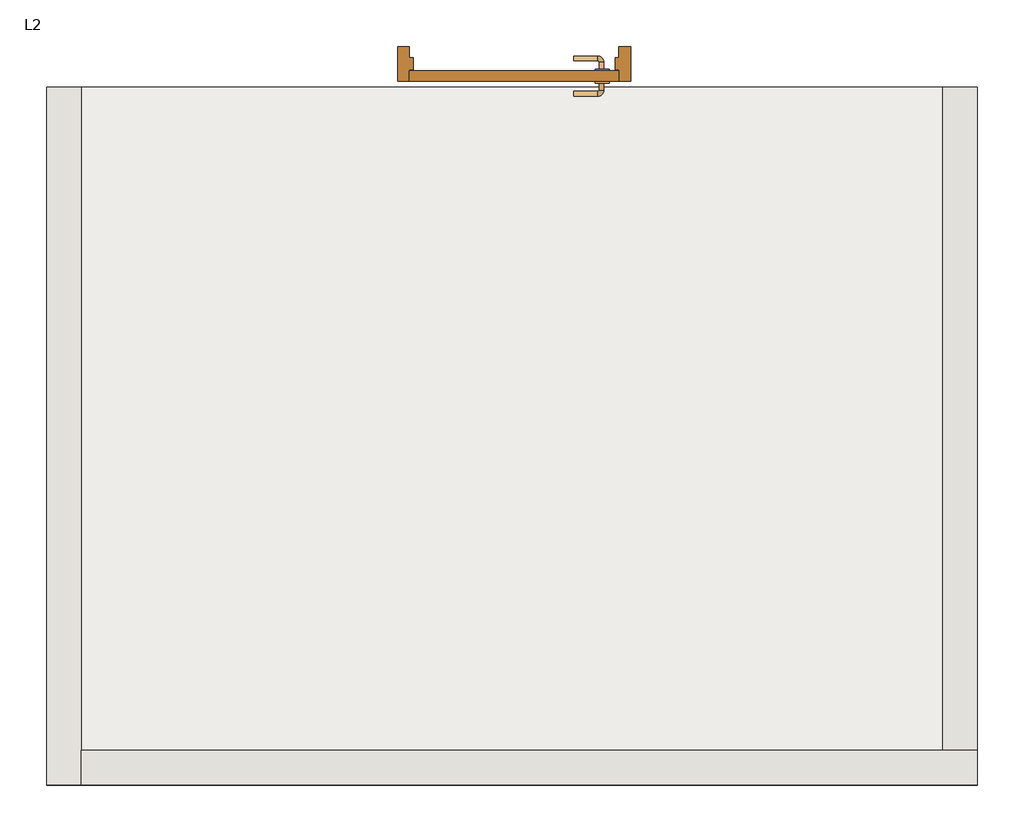
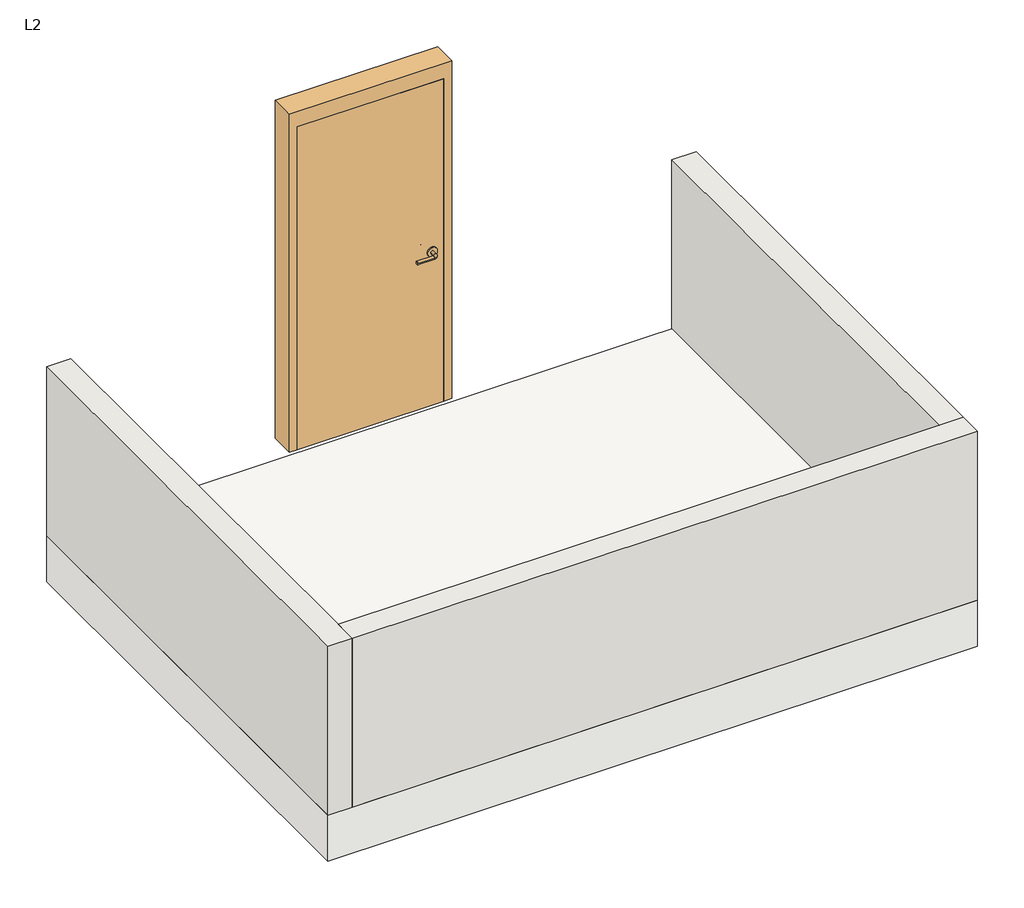
# One storey: 3 walls, 1 door, 1 slab.
"""IFC4 building model written with IfcOpenShell, lengths in millimetres."""

import ifcopenshell
import ifcopenshell.guid

model = None  # the IFC model being written
_history = None  # IfcOwnerHistory: only IFC2X3 demands one
_inside = {}  # id of a spatial element -> (the spatial element, [elements in it])
_under = {}  # id of a project, library or spatial element -> (it, [spatial elements below it])
_declared = {}  # id of a project -> (the project, [libraries it declares])
_typed = {}  # id of a type object -> (the type object, [elements of that type])
_made_of = {}  # id of a material, layer set ... -> (it, [elements and type objects made of it])


def new_model(schema):
    """Start an empty IFC model of exactly this schema.

    Asked for "IFC4X3", IfcOpenShell would pick the latest addendum, in which some entities
    have other attributes; the version numbers below select the first issue.
    IFC2X3 requires an IfcOwnerHistory on every rooted entity: one is made here for all.
    """
    global model, _history
    if schema == "IFC4X3":
        model = ifcopenshell.file(schema_version=(4, 3, 0, 0))
    else:
        model = ifcopenshell.file(schema=schema)
    _inside.clear()
    _under.clear()
    _declared.clear()
    _typed.clear()
    _made_of.clear()
    _history = None
    if model.schema == "IFC2X3":
        org = make("IfcOrganization", Name="unknown")
        user = make(
            "IfcPersonAndOrganization",
            ThePerson=make("IfcPerson", FamilyName="unknown"),
            TheOrganization=org,
        )
        app = make(
            "IfcApplication",
            ApplicationDeveloper=org,
            Version="unknown",
            ApplicationFullName="unknown",
            ApplicationIdentifier="unknown",
        )
        _history = make(
            "IfcOwnerHistory",
            OwningUser=user,
            OwningApplication=app,
            ChangeAction="ADDED",
            CreationDate=0,
        )
    return model


def make(cls, **values):
    """One entity of the class cls with the attributes given. An attribute that is None is left unset."""
    return model.create_entity(
        cls, **{name: value for name, value in values.items() if value is not None}
    )


def rooted(cls, **values):
    """An entity with a GlobalId (a new one), such as an element, a storey or a relation."""
    return make(cls, GlobalId=ifcopenshell.guid.new(), OwnerHistory=_history, **values)


def si_unit(unit_type, name, prefix=None):
    """IfcSIUnit, for example si_unit("LENGTHUNIT", "METRE", prefix="MILLI")."""
    return make("IfcSIUnit", UnitType=unit_type, Prefix=prefix, Name=name)


def assignment(units):
    """IfcUnitAssignment: the units of a project."""
    return None if units is None else make("IfcUnitAssignment", Units=units)


def point(xyz):
    """IfcCartesianPoint."""
    return None if xyz is None else make("IfcCartesianPoint", Coordinates=xyz)


def direction(xyz):
    """IfcDirection."""
    return None if xyz is None else make("IfcDirection", DirectionRatios=xyz)


def frame(location, z_axis=None, x_axis=None):
    """IfcAxis2Placement3D, a coordinate frame: its origin and axes. An axis left out is left unset."""
    return make(
        "IfcAxis2Placement3D",
        Location=point(location),
        Axis=direction(z_axis),
        RefDirection=direction(x_axis),
    )


def frame_2d(location, x_axis=None):
    """IfcAxis2Placement2D, a coordinate frame in the plane: its origin and x axis."""
    return make(
        "IfcAxis2Placement2D", Location=point(location), RefDirection=direction(x_axis)
    )


def origin():
    """The frame at (0, 0, 0) with its axes left unset."""
    return frame((0.0, 0.0, 0.0))


def origin_with_axes():
    """The frame at (0, 0, 0) with the z axis (0, 0, 1) and the x axis (1, 0, 0) written out."""
    return frame((0.0, 0.0, 0.0), z_axis=(0.0, 0.0, 1.0), x_axis=(1.0, 0.0, 0.0))


def place(relative_to, where):
    """IfcLocalPlacement: puts the frame where relative to a parent placement (None: the world)."""
    return make(
        "IfcLocalPlacement", PlacementRelTo=relative_to, RelativePlacement=where
    )


def context(
    kind, dimensions, precision=None, world=None, true_north=None, identifier=None
):
    """IfcGeometricRepresentationContext, for example the 3D "Model" context."""
    return make(
        "IfcGeometricRepresentationContext",
        ContextIdentifier=identifier,
        ContextType=kind,
        CoordinateSpaceDimension=dimensions,
        Precision=precision,
        WorldCoordinateSystem=world,
        TrueNorth=true_north,
    )


def project(units=None, contexts=None):
    """IfcProject with its units and contexts."""
    return rooted(
        "IfcProject",
        Name="project",
        RepresentationContexts=contexts,
        UnitsInContext=assignment(units),
    )


def spatial(cls, under=None, at=None, **own):
    """A site, building, storey or space (cls), placed at a placement, below another one or the project."""
    s = rooted(cls, ObjectPlacement=at, **own)
    if under is not None:
        _under.setdefault(under.id(), (under, []))[1].append(s)
    return s


def polyline(points):
    """IfcPolyline through the points."""
    return make("IfcPolyline", Points=[point(p) for p in points])


def circle_curve(where, radius):
    """IfcCircle in the frame where."""
    return make("IfcCircle", Position=where, Radius=radius)


def ellipse_curve(where, semi_axis1, semi_axis2):
    """IfcEllipse in the frame where."""
    return make(
        "IfcEllipse", Position=where, SemiAxis1=semi_axis1, SemiAxis2=semi_axis2
    )


def trimmed(basis, trim1, trim2, sense, master):
    """IfcTrimmedCurve: the piece of a basis curve between two trims."""
    return make(
        "IfcTrimmedCurve",
        BasisCurve=basis,
        Trim1=trim1,
        Trim2=trim2,
        SenseAgreement=sense,
        MasterRepresentation=master,
    )


def segment(curve, same_sense, transition):
    """IfcCompositeCurveSegment."""
    return make(
        "IfcCompositeCurveSegment",
        Transition=transition,
        SameSense=same_sense,
        ParentCurve=curve,
    )


def composite_curve(segments, self_intersect=None):
    """IfcCompositeCurve: segments joined end to end."""
    return make("IfcCompositeCurve", Segments=segments, SelfIntersect=self_intersect)


def outline(outer, holes=None, kind="AREA"):
    """IfcArbitraryClosedProfileDef: a profile drawn as a closed curve; with holes, ...WithVoids."""
    if holes is None:
        return make("IfcArbitraryClosedProfileDef", ProfileType=kind, OuterCurve=outer)
    return make(
        "IfcArbitraryProfileDefWithVoids",
        ProfileType=kind,
        OuterCurve=outer,
        InnerCurves=holes,
    )


def extrude(swept, where, along, depth):
    """IfcExtrudedAreaSolid: the profile swept, set in the frame where, extruded along a direction by depth."""
    return make(
        "IfcExtrudedAreaSolid",
        SweptArea=swept,
        Position=where,
        ExtrudedDirection=direction(along),
        Depth=depth,
    )


def faces_of(points, faces, orient=None, outer=None):
    """IfcFace entities. A face is a list of loops; a loop is a list of indices into points, from 0.

    orient and outer hold one flag for each loop. By default every Orientation is true, the
    first loop of a face is its IfcFaceOuterBound and the others are IfcFaceBound.
    """
    made = []
    for i, loops in enumerate(faces):
        bounds = []
        for j, loop in enumerate(loops):
            is_outer = j == 0 if outer is None else outer[i][j]
            bounds.append(
                make(
                    "IfcFaceOuterBound" if is_outer else "IfcFaceBound",
                    Bound=make("IfcPolyLoop", Polygon=[points[k] for k in loop]),
                    Orientation=True if orient is None else orient[i][j],
                )
            )
        made.append(make("IfcFace", Bounds=bounds))
    return made


def faceted_brep(points, faces, orient=None, outer=None, voids=None):
    """IfcFacetedBrep: a solid bounded by flat faces; with voids (closed shells), ...WithVoids."""
    shared = [point(p) for p in points]
    hull = make("IfcClosedShell", CfsFaces=faces_of(shared, faces, orient, outer))
    if voids is None:
        return make("IfcFacetedBrep", Outer=hull)
    return make(
        "IfcFacetedBrepWithVoids",
        Outer=hull,
        Voids=[
            make(cls, CfsFaces=faces_of(shared, fs, o, b)) for cls, fs, o, b in voids
        ],
    )


def shape(context_of_items, identifier, shape_type, items):
    """IfcShapeRepresentation: the items that make up one representation, for example the "Body"."""
    return make(
        "IfcShapeRepresentation",
        ContextOfItems=context_of_items,
        RepresentationIdentifier=identifier,
        RepresentationType=shape_type,
        Items=items,
    )


def source(mapping_origin, context_of_items, identifier, shape_type, items):
    """IfcRepresentationMap: a shape defined once, which mapped items show again and again."""
    return make(
        "IfcRepresentationMap",
        MappingOrigin=mapping_origin,
        MappedRepresentation=shape(context_of_items, identifier, shape_type, items),
    )


def transform(
    local_origin,
    x_axis=None,
    y_axis=None,
    z_axis=None,
    scale=None,
    scale2=None,
    scale3=None,
    uniform=True,
):
    """IfcCartesianTransformationOperator3D, or its non-uniform kind. x_axis, y_axis, z_axis: its Axis1, 2, 3."""
    if uniform:
        return make(
            "IfcCartesianTransformationOperator3D",
            Axis1=direction(x_axis),
            Axis2=direction(y_axis),
            LocalOrigin=point(local_origin),
            Scale=scale,
            Axis3=direction(z_axis),
        )
    return make(
        "IfcCartesianTransformationOperator3DnonUniform",
        Axis1=direction(x_axis),
        Axis2=direction(y_axis),
        LocalOrigin=point(local_origin),
        Scale=scale,
        Axis3=direction(z_axis),
        Scale2=scale2,
        Scale3=scale3,
    )


def mapped(mapping_source, mapping_target):
    """IfcMappedItem: shows the shape of a source again, moved by a transform."""
    return make(
        "IfcMappedItem", MappingSource=mapping_source, MappingTarget=mapping_target
    )


def made_of(thing, what):
    """Note that an element or type object is made of a material, layer set ...; save() writes the relation."""
    if what is not None:
        _made_of.setdefault(what.id(), (what, []))[1].append(thing)
    return thing


def element(
    cls,
    number,
    at=None,
    inside=None,
    cuts=None,
    type_object=None,
    material=None,
    context=None,
    identifier="Body",
    shape_type=None,
    held_by="IfcProductDefinitionShape",
    body=None,
    shapes=None,
    **own,
):
    """One element of the class cls, such as IfcWall. Its Tag is "e" and its number.

    at: its placement. inside: the storey or other place that contains it. cuts: it is an
    opening in that element (IfcRelVoidsElement). A single representation is given by context,
    identifier, shape_type and body (its items); several are given by shapes. held_by: the class
    of the entity that holds the representations. save() writes the other relations.
    """
    e = rooted(cls, Tag="e%d" % number, ObjectPlacement=at, **own)
    if body is not None:
        shapes = [shape(context, identifier, shape_type, body)]
    if shapes is not None:
        e.Representation = make(held_by, Representations=shapes)
    if inside is not None:
        _inside.setdefault(inside.id(), (inside, []))[1].append(e)
    if cuts is not None:
        rooted(
            "IfcRelVoidsElement", RelatingBuildingElement=cuts, RelatedOpeningElement=e
        )
    if type_object is not None:
        _typed.setdefault(type_object.id(), (type_object, []))[1].append(e)
    return made_of(e, material)


def aggregate(whole, parts):
    """IfcRelAggregates: a whole, such as a stair, and the parts it consists of."""
    return rooted("IfcRelAggregates", RelatingObject=whole, RelatedObjects=parts)


def save(model, path):
    """Write the relations noted so far, then the file.

    IfcRelAggregates (storeys below a building ...), IfcRelContainedInSpatialStructure (elements
    in a storey), IfcRelDefinesByType, IfcRelAssociatesMaterial and IfcRelDeclares: one each for
    every whole, place, type object, material and project.
    """
    for whole, parts in _under.values():
        aggregate(whole, parts)
    for where, things in _inside.values():
        rooted(
            "IfcRelContainedInSpatialStructure",
            RelatedElements=things,
            RelatingStructure=where,
        )
    for kind, things in _typed.values():
        rooted("IfcRelDefinesByType", RelatedObjects=things, RelatingType=kind)
    for what, things in _made_of.values():
        rooted("IfcRelAssociatesMaterial", RelatedObjects=things, RelatingMaterial=what)
    for by, libraries in _declared.values():
        rooted("IfcRelDeclares", RelatingContext=by, RelatedDefinitions=libraries)
    model.write(path)


def plane_surface(at):
    """IfcPlane: the flat surface through the origin of the frame at, square to its z axis."""
    return make("IfcPlane", Position=at)


def cylinder_surface(at, radius):
    """IfcCylindricalSurface: all points at the distance radius from the z axis of the frame at."""
    return make("IfcCylindricalSurface", Position=at, Radius=radius)


def revolved_surface(curve, axis_point, axis_direction):
    """IfcSurfaceOfRevolution: the curve turned about the line through axis_point along axis_direction."""
    return make(
        "IfcSurfaceOfRevolution",
        SweptCurve=make("IfcArbitraryOpenProfileDef", ProfileType="CURVE", Curve=curve),
        AxisPosition=make("IfcAxis1Placement", Location=point(axis_point), Axis=direction(axis_direction)),
    )


def advanced_brep(points, edges, surfaces, faces):
    """IfcAdvancedBrep: a solid bounded by faces that lie on surfaces and meet in shared edges.

    An edge is (start, end): straight between two places in points (the first is 0);
    or (start, end, curve); or (start, end, curve, False) where it runs against its curve.
    A face is (place in surfaces, loops), or (place, loops, False) where it looks against
    its surface's normal. A loop lists edges by number (the first is 1), with a minus sign
    where the edge is run from its end to its start. The first loop is the outer one.
    """
    corners = [point(p) for p in points]
    vertices = [make("IfcVertexPoint", VertexGeometry=c) for c in corners]
    made = []
    for start, end, *more in edges:
        made.append(
            make(
                "IfcEdgeCurve",
                EdgeStart=vertices[start],
                EdgeEnd=vertices[end],
                EdgeGeometry=more[0] if more else make("IfcPolyline", Points=[corners[start], corners[end]]),
                SameSense=more[1] if len(more) > 1 else True,
            )
        )
    hull = []
    for where, loops, *sense in faces:
        bounds = []
        for j, loop in enumerate(loops):
            ring = [make("IfcOrientedEdge", EdgeElement=made[abs(k) - 1], Orientation=k > 0) for k in loop]
            bounds.append(
                make(
                    "IfcFaceOuterBound" if j == 0 else "IfcFaceBound",
                    Bound=make("IfcEdgeLoop", EdgeList=ring),
                    Orientation=True,
                )
            )
        hull.append(make("IfcAdvancedFace", Bounds=bounds, FaceSurface=surfaces[where], SameSense=sense[0] if sense else True))
    return make("IfcAdvancedBrep", Outer=make("IfcClosedShell", CfsFaces=hull))


def m_door_passage_single_flush_900_x_2100mm_f70d95c9(model_context):
    return source(origin(), model_context, "Body", "SolidModel", [
        advanced_brep(
        [(-384.990625, 3.35, 1000.0), (-364.990625, 3.35, 1000.0), (-364.990625, -26.65, 1000.0), (-384.990625, -26.65, 1000.0), (-359.990625, -31.65, 1000.0), (-359.990625, -51.65, 1000.0), (-254.990625, -51.65, 1000.0), (-254.990625, -31.65, 1000.0)],
        [
            (0, 1, circle_curve(frame((-374.990625, 3.35, 1000.0), z_axis=(0.0, 1.0, 0.0), x_axis=(1.0, 0.0, 0.0)), 10.0)),
            (1, 0, circle_curve(frame((-374.990625, 3.35, 1000.0), z_axis=(0.0, 1.0, 0.0), x_axis=(1.0, 0.0, 0.0)), 10.0)),
            (1, 2),
            (2, 3, circle_curve(frame((-374.990625, -26.65, 1000.0), z_axis=(0.0, 1.0, 0.0), x_axis=(1.0, 0.0, 0.0)), 10.0)),
            (3, 0),
            (3, 2, circle_curve(frame((-374.990625, -26.65, 1000.0), z_axis=(0.0, 1.0, 0.0), x_axis=(1.0, 0.0, 0.0)), 10.0)),
            (4, 5, circle_curve(frame((-359.990625, -41.65, 1000.0), z_axis=(-1.0, 0.0, 0.0), x_axis=(0.0, 1.0, 0.0)), 10.0)),
            (5, 3, circle_curve(frame((-359.990625, -26.65, 1000.0), z_axis=(0.0, 0.0, -1.0), x_axis=(-1.0, 0.0, 0.0)), 25.0)),
            (2, 4, circle_curve(frame((-359.990625, -26.65, 1000.0), z_axis=(0.0, 0.0, 1.0), x_axis=(-1.0, 0.0, 0.0)), 5.0)),
            (5, 4, circle_curve(frame((-359.990625, -41.65, 1000.0), z_axis=(-1.0, 0.0, 0.0), x_axis=(0.0, 1.0, 0.0)), 10.0)),
            (6, 7, circle_curve(frame((-254.990625, -41.65, 1000.0), z_axis=(1.0, 0.0, 0.0), x_axis=(0.0, 1.0, 0.0)), 10.0)),
            (7, 6, circle_curve(frame((-254.990625, -41.65, 1000.0), z_axis=(1.0, 0.0, 0.0), x_axis=(0.0, 1.0, 0.0)), 10.0)),
            (4, 7),
            (6, 5),
        ],
        [
            plane_surface(frame((-374.990625, 3.35, 1000.0), z_axis=(0.0, 1.0, 0.0), x_axis=(0.0, 0.0, 1.0))),
            cylinder_surface(frame((-374.990625, 3.35, 1000.0), z_axis=(0.0, 1.0, 0.0), x_axis=(1.0, 0.0, 0.0)), 10.0),
            revolved_surface(trimmed(ellipse_curve(frame((-374.990625, -26.65, 1000.0), z_axis=(0.0, -1.0, 0.0), x_axis=(1.0, 0.0, 0.0)), 10.0, 10.0), [point((-384.990625, -26.65, 1000.0))], [point((-364.990625, -26.65, 1000.0))], True, "CARTESIAN"), (-359.990625, -26.65, 1000.0), (0.0, 0.0, -1.0)),
            revolved_surface(trimmed(ellipse_curve(frame((-374.990625, -26.65, 1000.0), z_axis=(0.0, -1.0, 0.0), x_axis=(1.0, 0.0, 0.0)), 10.0, 10.0), [point((-364.990625, -26.65, 1000.0))], [point((-384.990625, -26.65, 1000.0))], True, "CARTESIAN"), (-359.990625, -26.65, 1000.0), (0.0, 0.0, -1.0)),
            plane_surface(frame((-254.990625, -41.65, 1000.0), z_axis=(1.0, 0.0, 0.0), x_axis=(0.0, 0.0, 1.0))),
            cylinder_surface(frame((-359.990625, -41.65, 1000.0), z_axis=(-1.0, 0.0, 0.0), x_axis=(0.0, 1.0, 0.0)), 10.0),
        ],
        [
            (0, [[1, 2]]),
            (1, [[3, 4, 5, -2]]),
            (1, [[-5, 6, -3, -1]]),
            (2, [[7, 8, -4, 9]]),
            (3, [[10, -9, -6, -8]]),
            (4, [[11, 12]]),
            (5, [[13, -11, 14, -7]]),
            (5, [[-14, -12, -13, -10]]),
        ],
    ),
        extrude(outline(composite_curve([segment(trimmed(circle_curve(frame_2d((1000.0, -377.490625)), 30.0), [point((1000.0, -407.490625))], [point((1000.0, -347.490625))], False, "CARTESIAN"), True, "CONTINUOUS"), segment(trimmed(circle_curve(frame_2d((1000.0, -377.490625)), 30.0), [point((1000.0, -347.490625))], [point((1000.0, -407.490625))], False, "CARTESIAN"), True, "CONTINUOUS")], self_intersect=False)), frame((0.0, 3.35, 0.0), z_axis=(0.0, 1.0, 0.0), x_axis=(0.0, 0.0, 1.0)), (0.0, 0.0, 1.0), 8.0),
        advanced_brep(
        [(-384.990625, 64.35, 1000.0), (-364.990625, 64.35, 1000.0), (-384.990625, 94.35, 1000.0), (-364.990625, 94.35, 1000.0), (-359.990625, 99.35, 1000.0), (-359.990625, 119.35, 1000.0), (-254.990625, 119.35, 1000.0), (-254.990625, 99.35, 1000.0)],
        [
            (0, 1, circle_curve(frame((-374.990625, 64.35, 1000.0), z_axis=(0.0, -1.0, 0.0), x_axis=(1.0, 0.0, 0.0)), 10.0)),
            (1, 0, circle_curve(frame((-374.990625, 64.35, 1000.0), z_axis=(0.0, -1.0, 0.0), x_axis=(1.0, 0.0, 0.0)), 10.0)),
            (0, 2),
            (2, 3, circle_curve(frame((-374.990625, 94.35, 1000.0), z_axis=(0.0, -1.0, 0.0), x_axis=(1.0, 0.0, 0.0)), 10.0)),
            (3, 1),
            (3, 2, circle_curve(frame((-374.990625, 94.35, 1000.0), z_axis=(0.0, -1.0, 0.0), x_axis=(1.0, 0.0, 0.0)), 10.0)),
            (4, 3, circle_curve(frame((-359.990625, 94.35, 1000.0), z_axis=(0.0, 0.0, 1.0), x_axis=(-1.0, 0.0, 0.0)), 5.0)),
            (2, 5, circle_curve(frame((-359.990625, 94.35, 1000.0), z_axis=(0.0, 0.0, -1.0), x_axis=(-1.0, 0.0, 0.0)), 25.0)),
            (5, 4, circle_curve(frame((-359.990625, 109.35, 1000.0), z_axis=(-1.0, 0.0, 0.0), x_axis=(0.0, -1.0, 0.0)), 10.0)),
            (4, 5, circle_curve(frame((-359.990625, 109.35, 1000.0), z_axis=(-1.0, 0.0, 0.0), x_axis=(0.0, -1.0, 0.0)), 10.0)),
            (6, 7, circle_curve(frame((-254.990625, 109.35, 1000.0), z_axis=(1.0, 0.0, 0.0), x_axis=(0.0, -1.0, 0.0)), 10.0)),
            (7, 6, circle_curve(frame((-254.990625, 109.35, 1000.0), z_axis=(1.0, 0.0, 0.0), x_axis=(0.0, -1.0, 0.0)), 10.0)),
            (5, 6),
            (7, 4),
        ],
        [
            plane_surface(frame((-374.990625, 64.35, 1000.0), z_axis=(0.0, -1.0, 0.0), x_axis=(0.0, 0.0, 1.0))),
            cylinder_surface(frame((-374.990625, 64.35, 1000.0), z_axis=(0.0, -1.0, 0.0), x_axis=(1.0, 0.0, 0.0)), 10.0),
            revolved_surface(trimmed(ellipse_curve(frame((-374.990625, 94.35, 1000.0), z_axis=(0.0, -1.0, 0.0), x_axis=(1.0, 0.0, 0.0)), 10.0, 10.0), [point((-384.990625, 94.35, 1000.0))], [point((-364.990625, 94.35, 1000.0))], True, "CARTESIAN"), (-359.990625, 94.35, 1000.0), (0.0, 0.0, -1.0)),
            revolved_surface(trimmed(ellipse_curve(frame((-374.990625, 94.35, 1000.0), z_axis=(0.0, -1.0, 0.0), x_axis=(1.0, 0.0, 0.0)), 10.0, 10.0), [point((-364.990625, 94.35, 1000.0))], [point((-384.990625, 94.35, 1000.0))], True, "CARTESIAN"), (-359.990625, 94.35, 1000.0), (0.0, 0.0, -1.0)),
            plane_surface(frame((-254.990625, 109.35, 1000.0), z_axis=(1.0, 0.0, 0.0), x_axis=(0.0, 0.0, 1.0))),
            cylinder_surface(frame((-359.990625, 109.35, 1000.0), z_axis=(-1.0, 0.0, 0.0), x_axis=(0.0, -1.0, 0.0)), 10.0),
        ],
        [
            (0, [[1, 2]]),
            (1, [[-1, 3, 4, 5]]),
            (1, [[-2, -5, 6, -3]]),
            (2, [[7, -4, 8, 9]]),
            (3, [[-8, -6, -7, 10]]),
            (4, [[11, 12]]),
            (5, [[-9, 13, -12, 14]]),
            (5, [[-10, -14, -11, -13]]),
        ],
    ),
        extrude(outline(composite_curve([segment(trimmed(circle_curve(frame_2d((1000.0, -377.490625)), 30.0), [point((1000.0, -407.490625))], [point((1000.0, -347.490625))], False, "CARTESIAN"), True, "CONTINUOUS"), segment(trimmed(circle_curve(frame_2d((1000.0, -377.490625)), 30.0), [point((1000.0, -347.490625))], [point((1000.0, -407.490625))], False, "CARTESIAN"), True, "CONTINUOUS")], self_intersect=False)), frame((0.0, 56.35, 0.0), z_axis=(0.0, 1.0, 0.0), x_axis=(0.0, 0.0, 1.0)), (0.0, 0.0, 1.0), 8.0),
        extrude(outline(polyline([(450.0, 11.35), (-450.0, 11.35), (-450.0, 56.35), (450.0, 56.35), (450.0, 11.35)])), origin_with_axes(), (0.0, 0.0, 1.0), 2100.0),
        faceted_brep([(450.0, 6.5875, 0.0), (450.0, 56.35, 0.0), (500.0, 56.35, 0.0), (500.0, -93.65, 0.0), (450.0, -93.65, 0.0), (450.0, -44.4375, 0.0), (434.125, -44.4375, 0.0), (434.125, 6.5875, 0.0), (450.0, 6.5875, 2100.0), (450.0, 56.35, 2100.0), (-450.0, 56.35, 2100.0), (-450.0, 56.35, 0.0), (-500.0, 56.35, 0.0), (-500.0, 56.35, 2200.0), (500.0, 56.35, 2200.0), (500.0, -93.65, 2200.0), (-500.0, -93.65, 2200.0), (-500.0, -93.65, 0.0), (-450.0, -93.65, 0.0), (-450.0, -93.65, 2100.0), (450.0, -93.65, 2100.0), (450.0, -44.4375, 2100.0), (-450.0, -44.4375, 2100.0), (-450.0, -44.4375, 0.0), (-434.125, -44.4375, 0.0), (-434.125, -44.4375, 2084.125), (434.125, -44.4375, 2084.125), (434.125, 6.5875, 2084.125), (-434.125, 6.5875, 2084.125), (-434.125, 6.5875, 0.0), (-450.0, 6.5875, 0.0), (-450.0, 6.5875, 2100.0)], [[[0, 1, 2, 3, 4, 5, 6, 7]], [[1, 0, 8, 9]], [[2, 1, 9, 10, 11, 12, 13, 14]], [[3, 2, 14, 15]], [[4, 3, 15, 16, 17, 18, 19, 20]], [[5, 4, 20, 21]], [[6, 5, 21, 22, 23, 24, 25, 26]], [[7, 6, 26, 27]], [[0, 7, 27, 28, 29, 30, 31, 8]], [[9, 8, 31, 10]], [[20, 19, 22, 21]], [[26, 25, 28, 27]], [[12, 11, 30, 29, 24, 23, 18, 17]], [[11, 10, 31, 30]], [[13, 12, 17, 16]], [[19, 18, 23, 22]], [[25, 24, 29, 28]], [[15, 14, 13, 16]]]),
    ])


model = new_model("IFC4")

# Units and contexts
model_context = context("Model", 3, world=origin())
ifc_project = project(units=[si_unit("LENGTHUNIT", "METRE", prefix="MILLI")], contexts=[model_context])

# Site, building, storey
site = spatial("IfcSite", under=ifc_project)
building = spatial("IfcBuilding", under=site)
storey = spatial("IfcBuildingStorey", under=building, Name="L2", Elevation=1200.0)

# Door
placement = place(None, origin())
m_door_passage_single_flush_900_x_2100mm_shape = m_door_passage_single_flush_900_x_2100mm_f70d95c9(model_context)
element("IfcDoor", 1, ObjectType="M_Door-Passage-Single-Flush : 900 x 2100mm", at=placement, inside=storey, context=model_context, shape_type="MappedRepresentation", body=[
    mapped(m_door_passage_single_flush_900_x_2100mm_shape, transform((752.7568, 2222.9207088, 1200.0), x_axis=(-1.0, 0.0, 0.0), y_axis=(0.0, -1.0, 0.0), z_axis=(0.0, 0.0, 1.0))),
])

# Slab
element("IfcSlab", 2, ObjectType="Generic 300mm", at=placement, inside=storey, context=model_context, shape_type="SweptSolid", body=[
    extrude(outline(polyline([(2743.2318, -858.4292912), (-1256.7682, -858.4292912), (-1256.7682, 2141.5707088), (2743.2318, 2141.5707088), (2743.2318, -858.4292912)])), frame((0.0, 0.0, 900.0), z_axis=(0.0, 0.0, 1.0), x_axis=(1.0, 0.0, 0.0)), (0.0, 0.0, 1.0), 300.0),
])

# Walls
element("IfcWall", 3, ObjectType="Generic - 150mm", at=placement, inside=storey, context=model_context, shape_type="Brep", body=[
    faceted_brep([(-1256.7682, 2141.5707088, 1200.0), (-1256.7682, -858.4292912, 1200.0), (-1256.7682, -858.4292912, 2300.0), (-1256.7682, 2141.5707088, 2300.0), (-1106.7682, 2141.5707088, 1200.0), (-1106.7682, 2141.5707088, 2300.0), (-1106.7682, -708.4292912, 2300.0), (-1106.7682, -858.4292912, 2300.0), (-1106.7682, -858.4292912, 1200.0), (-1106.7682, -708.4292912, 1200.0)], [[[0, 1, 2, 3]], [[4, 5, 6, 7, 8, 9]], [[1, 0, 4, 9, 8]], [[3, 2, 7, 6, 5]], [[0, 3, 5, 4]], [[2, 1, 8, 7]]]),
])
element("IfcWall", 4, ObjectType="Generic - 150mm", at=placement, inside=storey, context=model_context, shape_type="Brep", body=[
    faceted_brep([(-1106.7682, -858.4292912, 1200.0), (2743.2318, -858.4292912, 1200.0), (2743.2318, -858.4292912, 2300.0), (-1106.7682, -858.4292912, 2300.0), (-1106.7682, -708.4292912, 1200.0), (-1106.7682, -708.4292912, 2300.0), (2593.2318, -708.4292912, 2300.0), (2743.2318, -708.4292912, 2300.0), (2743.2318, -708.4292912, 1200.0), (2593.2318, -708.4292912, 1200.0)], [[[0, 1, 2, 3]], [[4, 5, 6, 7, 8, 9]], [[1, 0, 4, 9, 8]], [[3, 2, 7, 6, 5]], [[0, 3, 5, 4]], [[2, 1, 8, 7]]]),
])
element("IfcWall", 5, ObjectType="Generic - 150mm", at=placement, inside=storey, context=model_context, shape_type="SweptSolid", body=[
    extrude(outline(polyline([(2743.2318, 2141.5707088), (2743.2318, -708.4292912), (2593.2318, -708.4292912), (2593.2318, 2141.5707088), (2743.2318, 2141.5707088)])), frame((0.0, 0.0, 1200.0), z_axis=(0.0, 0.0, 1.0), x_axis=(1.0, 0.0, 0.0)), (0.0, 0.0, 1.0), 1100.0),
])

save(model, "model.ifc")

# Revit data of these elements
# Type "M_Door-Passage-Single-Flush : 900 x 2100mm"
#   Type Mark = "38"
#   Analytic Construction = "Wooden"
#   Thickness = 45 mm
#   Thermal Resistance (R) = 0.455703 (m²·K)/W
#   Swing Angle [instance default] = 90.00°
#   Strike Height = 1000 mm
#   Rough Width [instance default] = 1000 mm
#   Rough Height [instance default] = 2200 mm
#   MF Opening Height [instance default] = 100 mm
#   MF Opening Width [instance default] = 100 mm
#   Inset Calculate [instance default] = 105 mm
#   Masonry Inset [instance default] = 25 mm
#   Height = 2100 mm
#   Width = 900 mm
#   Heat Transfer Coefficient (U) = 2.19465 W/(m²·K)
#   Masonry Frame Depth = 150 mm
#   Masonry Frame [instance default] = yes
#   Function = 1
#   Dry Wall Frame [instance default] = no
#   Panel Material = Wood - Birch
#   Frame Material = Metal - Paint Finish - Grey
#   Door Handle Material = Aluminum
#   Visual Light Transmittance = 0
#   Solar Heat Gain Coefficient = 0
#   Wall Closure = (empty or 0)
# Type "Generic 300mm"
#   Description = "Generic Floor (Material By Category), 300mm thick"
#   Function = 0
#   Layers, outside or top first: 300 mm no material (function 1)
# Type "Generic - 150mm"
#   Description = "Generic Wall (Material By Category), 150mm thick"
#   Type Mark = "G04"
#   Layers, outside or top first: 150 mm no material (function 1)
# Element 1 (IfcDoor, "M_Door-Passage-Single-Flush : 900 x 2100mm")
#   Swing Angle = 90.00°
#   Rough Width = 1000 mm
#   Rough Height = 2200 mm
#   Masonry Inset = 25 mm
#   MF Opening Width = 100 mm
#   MF Opening Height = 100 mm
#   Inset Calculate = 105 mm
#   Masonry Frame = yes
#   Dry Wall Frame = no
#   Phase Created = New Construction
#   Materials on its faces: "Aluminum", "Metal - Paint Finish - Grey", "Wood - Birch"
# Element 2 (IfcSlab, "Generic 300mm")
#   Height Offset From Level = 0 mm
#   Phase Created = New Construction
#   Materials on its faces: "Default Floor"
# Elements 3, 4, 5 (IfcWall, "Generic - 150mm")
#   Top Offset = 0 mm
#   Base Offset = 0 mm
#   Unconnected Height = 1100 mm
#   wall height = 1100 mm
#   Phase Created = New Construction
#   Base Constraint = L2
#   Materials on its faces: "Default Wall"
# Materials
#   "Wood - Birch": class "Wood", colour RGB 173 132 96, transparency 0, Cost = 0
#   "Metal - Paint Finish - Grey": class "Paint", colour RGB 178 178 178, transparency 0, Cost = 0
#   "Aluminum": class "Metal", colour RGB 244 245 246, transparency 0, Description = "Aluminum 6061", Cost = 0
#   "Default Floor": class "Miscellaneous", colour RGB 128 128 128, transparency 0, Cost = 0
#   "Default Wall": class "Miscellaneous", colour RGB 192 192 192, transparency 0, Cost = 0
